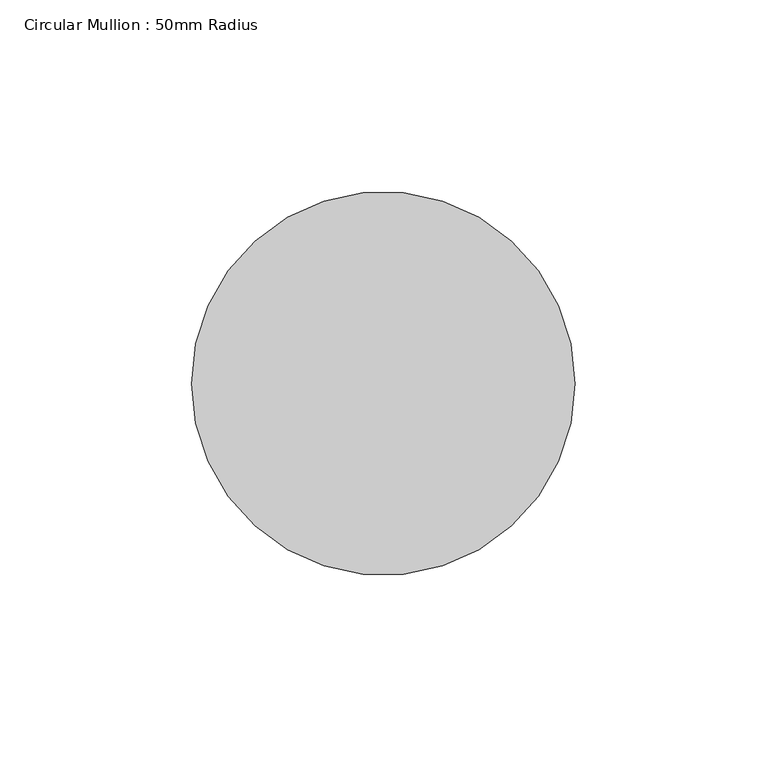
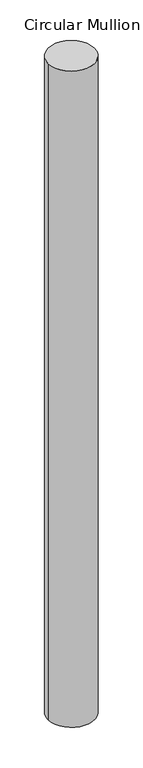
"""IFC4 building model written with IfcOpenShell, lengths in millimetres: member geometry, Circular Mullion : 50mm Radius."""

from ifc_helpers import new_model, si_unit, point, frame, origin, origin_2d, place, context, project, spatial, circle_curve, trimmed, segment, composite_curve, outline, extrude, source, transform, mapped, element, save


def circular_mullion_50mm_radius_086751e1(model_context):
    return source(origin(), model_context, "Body", "SweptSolid", [
        extrude(outline(composite_curve([segment(trimmed(circle_curve(origin_2d(), 50.0), [point((50.0, 0.0))], [point((-50.0, 0.0))], False, "CARTESIAN"), True, "CONTINUOUS"), segment(trimmed(circle_curve(origin_2d(), 50.0), [point((-50.0, 0.0))], [point((50.0, 0.0))], False, "CARTESIAN"), True, "CONTINUOUS")], self_intersect=False)), frame((0.0, 0.0, -1492.971844), z_axis=(0.0, 0.0, 1.0), x_axis=(1.0, 0.0, 0.0)), (0.0, 0.0, 1.0), 1492.971844),
    ])


if __name__ == "__main__":
    model = new_model("IFC4")
    model_context = context("Model", 3, world=origin())
    ifc_project = project(units=[si_unit("LENGTHUNIT", "METRE", prefix="MILLI")], contexts=[model_context])
    site = spatial("IfcSite", under=ifc_project)
    building = spatial("IfcBuilding", under=site)
    placement = place(None, origin())
    circular_mullion_50mm_radius_shape = circular_mullion_50mm_radius_086751e1(model_context)
    element("IfcMember", 1, ObjectType="Circular Mullion : 50mm Radius", at=placement, inside=building, context=model_context, shape_type="MappedRepresentation", body=[
        mapped(circular_mullion_50mm_radius_shape, transform((0.0, 0.0, 0.0), x_axis=(1.0, 0.0, 0.0), y_axis=(0.0, 1.0, 0.0), z_axis=(0.0, 0.0, 1.0))),
    ])
    save(model, "model.ifc")

# Revit data of these elements
# Type "Circular Mullion : 50mm Radius"
#   built-in parameter 1007350 = 0.164042 (stored number, unit not read)
# Element 1 (IfcMember, "Circular Mullion : 50mm Radius")
#   Materials on its faces: "Aluminium"
# Materials
#   "Aluminium": class "Metal", colour RGB 247 247 247, transparency 0, Description = "Aluminium 6061", Cost = 0
